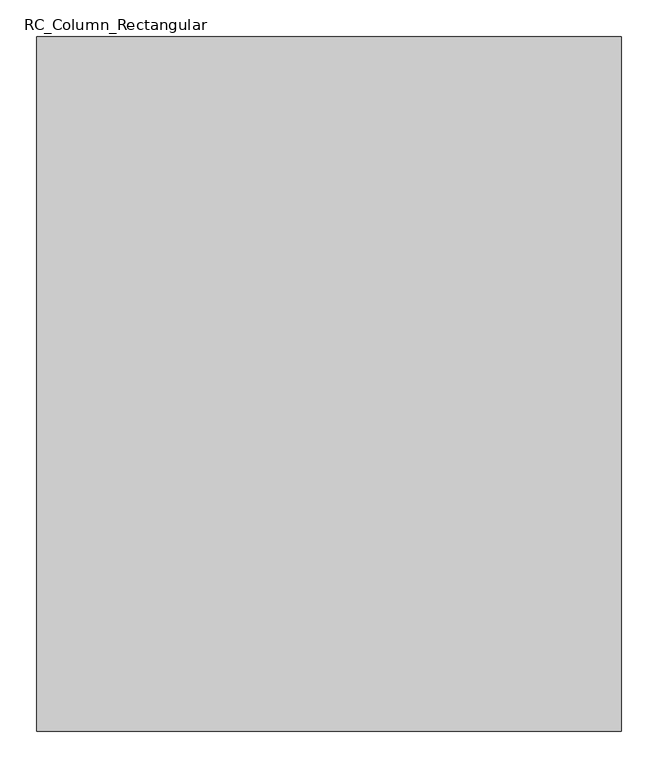
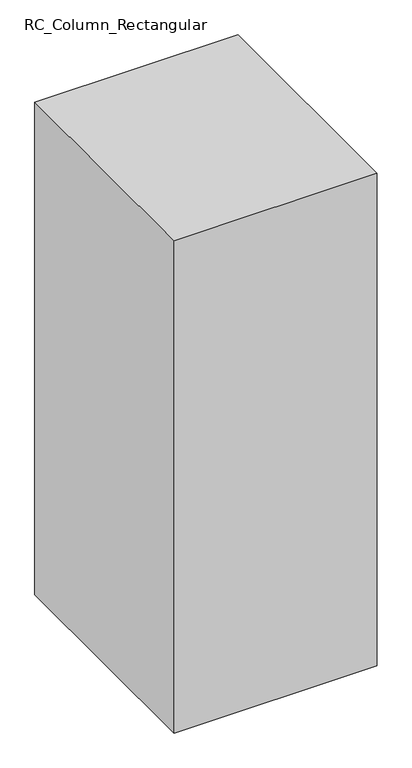
"""IFC4 building model written with IfcOpenShell, lengths in millimetres: column geometry, RC_Column_Rectangular : H_SC_AR_S15_UG PED_W800xL950_Bit_PD1."""

from ifc_helpers import new_model, si_unit, frame, origin, place, context, project, spatial, polyline, outline, extrude, source, transform, mapped, element, save


def rc_column_rectangular_8fcc3407(model_context):
    return source(origin(), model_context, "Body", "SweptSolid", [
        extrude(outline(polyline([(400.0, 475.0), (400.0, -475.0), (-400.0, -475.0), (-400.0, 475.0), (400.0, 475.0)])), frame((0.0, 0.0, -9380.1756499), z_axis=(0.0, 0.0, 1.0), x_axis=(1.0, 0.0, 0.0)), (0.0, 0.0, 1.0), 2050.0),
    ])


if __name__ == "__main__":
    model = new_model("IFC4")
    model_context = context("Model", 3, world=origin())
    ifc_project = project(units=[si_unit("LENGTHUNIT", "METRE", prefix="MILLI")], contexts=[model_context])
    site = spatial("IfcSite", under=ifc_project)
    building = spatial("IfcBuilding", under=site)
    placement = place(None, origin())
    rc_column_rectangular_shape = rc_column_rectangular_8fcc3407(model_context)
    element("IfcColumn", 1, ObjectType="RC_Column_Rectangular : H_SC_AR_S15_UG PED_W800xL950_Bit_PD1", at=placement, inside=building, context=model_context, shape_type="MappedRepresentation", body=[
        mapped(rc_column_rectangular_shape, transform((0.0, 0.0, 0.0), x_axis=(1.0, 0.0, 0.0), y_axis=(0.0, 1.0, 0.0), z_axis=(0.0, 0.0, 1.0))),
    ])
    save(model, "model.ifc")

# Revit data of these elements
# Type "RC_Column_Rectangular : H_SC_AR_S15_UG PED_W800xL950_Bit_PD1"
#   Type Mark = "PD1"
#   Width = 800 mm
#   Length = 950 mm
#   hec_material3 [instance default] = none
#   hec_material2 [instance default] = none
#   hec_material1 [instance default] = none
#   Structural Material [instance default] = none
#   Description = (empty or 0)
